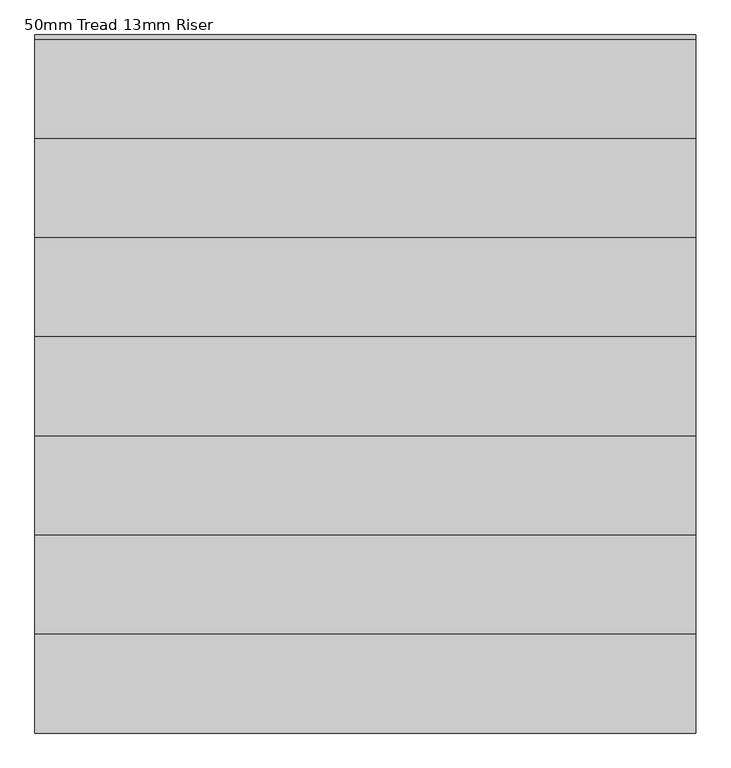
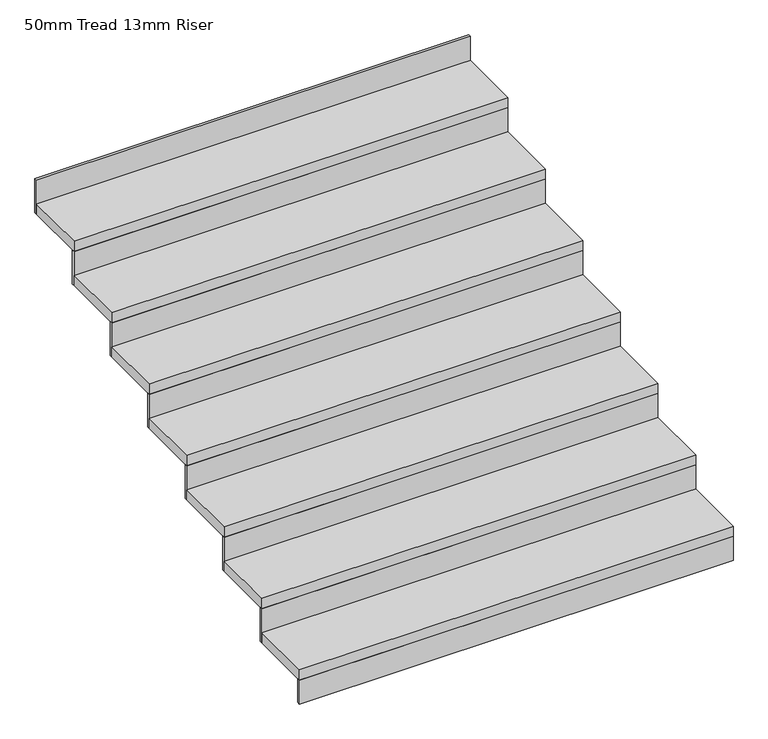
"""IFC4 building model written with IfcOpenShell, lengths in millimetres: stair flight geometry, 50mm Tread 13mm Riser."""

from ifc_helpers import new_model, si_unit, frame, origin, place, context, project, spatial, polyline, outline, extrude, source, transform, mapped, element, save


def stair_flight_50mm_tread_13mm_riser_f0df06f7(model_context):
    return source(origin(), model_context, "Body", "SweptSolid", [
        extrude(outline(polyline([(14700.0002443, 21382.4999999), (14700.0002443, 21369.9999999), (12700.0002443, 21369.9999999), (12700.0002443, 21382.4999999), (14700.0002443, 21382.4999999)])), frame((0.0, 0.0, 26500.0), z_axis=(0.0, 0.0, 1.0), x_axis=(1.0, 0.0, 0.0)), (0.0, 0.0, 1.0), 116.6666667),
        extrude(outline(polyline([(12700.0002443, 21669.9999999), (14700.0002443, 21669.9999999), (14700.0002443, 21369.9999999), (12700.0002443, 21369.9999999), (12700.0002443, 21669.9999999)])), frame((0.0, 0.0, 26616.6666667), z_axis=(0.0, 0.0, 1.0), x_axis=(1.0, 0.0, 0.0)), (0.0, 0.0, 1.0), 50.0),
        extrude(outline(polyline([(14700.0002443, 21682.4999999), (14700.0002443, 21669.9999999), (12700.0002443, 21669.9999999), (12700.0002443, 21682.4999999), (14700.0002443, 21682.4999999)])), frame((0.0, 0.0, 26616.6666667), z_axis=(0.0, 0.0, 1.0), x_axis=(1.0, 0.0, 0.0)), (0.0, 0.0, 1.0), 166.6666667),
        extrude(outline(polyline([(12700.0002443, 21969.9999999), (14700.0002443, 21969.9999999), (14700.0002443, 21669.9999999), (12700.0002443, 21669.9999999), (12700.0002443, 21969.9999999)])), frame((0.0, 0.0, 26783.3333333), z_axis=(0.0, 0.0, 1.0), x_axis=(1.0, 0.0, 0.0)), (0.0, 0.0, 1.0), 50.0),
        extrude(outline(polyline([(14700.0002443, 21982.4999999), (14700.0002443, 21969.9999999), (12700.0002443, 21969.9999999), (12700.0002443, 21982.4999999), (14700.0002443, 21982.4999999)])), frame((0.0, 0.0, 26783.3333333), z_axis=(0.0, 0.0, 1.0), x_axis=(1.0, 0.0, 0.0)), (0.0, 0.0, 1.0), 166.6666667),
        extrude(outline(polyline([(12700.0002443, 22269.9999999), (14700.0002443, 22269.9999999), (14700.0002443, 21969.9999999), (12700.0002443, 21969.9999999), (12700.0002443, 22269.9999999)])), frame((0.0, 0.0, 26950.0), z_axis=(0.0, 0.0, 1.0), x_axis=(1.0, 0.0, 0.0)), (0.0, 0.0, 1.0), 50.0),
        extrude(outline(polyline([(14700.0002443, 22282.4999999), (14700.0002443, 22269.9999999), (12700.0002443, 22269.9999999), (12700.0002443, 22282.4999999), (14700.0002443, 22282.4999999)])), frame((0.0, 0.0, 26950.0), z_axis=(0.0, 0.0, 1.0), x_axis=(1.0, 0.0, 0.0)), (0.0, 0.0, 1.0), 166.6666667),
        extrude(outline(polyline([(12700.0002443, 22569.9999999), (14700.0002443, 22569.9999999), (14700.0002443, 22269.9999999), (12700.0002443, 22269.9999999), (12700.0002443, 22569.9999999)])), frame((0.0, 0.0, 27116.6666667), z_axis=(0.0, 0.0, 1.0), x_axis=(1.0, 0.0, 0.0)), (0.0, 0.0, 1.0), 50.0),
        extrude(outline(polyline([(14700.0002443, 22582.4999999), (14700.0002443, 22569.9999999), (12700.0002443, 22569.9999999), (12700.0002443, 22582.4999999), (14700.0002443, 22582.4999999)])), frame((0.0, 0.0, 27116.6666667), z_axis=(0.0, 0.0, 1.0), x_axis=(1.0, 0.0, 0.0)), (0.0, 0.0, 1.0), 166.6666667),
        extrude(outline(polyline([(12700.0002443, 22869.9999999), (14700.0002443, 22869.9999999), (14700.0002443, 22569.9999999), (12700.0002443, 22569.9999999), (12700.0002443, 22869.9999999)])), frame((0.0, 0.0, 27283.3333333), z_axis=(0.0, 0.0, 1.0), x_axis=(1.0, 0.0, 0.0)), (0.0, 0.0, 1.0), 50.0),
        extrude(outline(polyline([(14700.0002443, 22882.4999999), (14700.0002443, 22869.9999999), (12700.0002443, 22869.9999999), (12700.0002443, 22882.4999999), (14700.0002443, 22882.4999999)])), frame((0.0, 0.0, 27283.3333333), z_axis=(0.0, 0.0, 1.0), x_axis=(1.0, 0.0, 0.0)), (0.0, 0.0, 1.0), 166.6666667),
        extrude(outline(polyline([(12700.0002443, 23169.9999999), (14700.0002443, 23169.9999999), (14700.0002443, 22869.9999999), (12700.0002443, 22869.9999999), (12700.0002443, 23169.9999999)])), frame((0.0, 0.0, 27450.0), z_axis=(0.0, 0.0, 1.0), x_axis=(1.0, 0.0, 0.0)), (0.0, 0.0, 1.0), 50.0),
        extrude(outline(polyline([(14700.0002443, 23182.4999999), (14700.0002443, 23169.9999999), (12700.0002443, 23169.9999999), (12700.0002443, 23182.4999999), (14700.0002443, 23182.4999999)])), frame((0.0, 0.0, 27450.0), z_axis=(0.0, 0.0, 1.0), x_axis=(1.0, 0.0, 0.0)), (0.0, 0.0, 1.0), 166.6666667),
        extrude(outline(polyline([(14700.0002443, 23482.4999999), (14700.0002443, 23469.9999999), (12700.0002443, 23469.9999999), (12700.0002443, 23482.4999999), (14700.0002443, 23482.4999999)])), frame((0.0, 0.0, 27616.6666667), z_axis=(0.0, 0.0, 1.0), x_axis=(1.0, 0.0, 0.0)), (0.0, 0.0, 1.0), 166.6666667),
        extrude(outline(polyline([(12700.0002443, 23469.9999999), (14700.0002443, 23469.9999999), (14700.0002443, 23169.9999999), (12700.0002443, 23169.9999999), (12700.0002443, 23469.9999999)])), frame((0.0, 0.0, 27616.6666667), z_axis=(0.0, 0.0, 1.0), x_axis=(1.0, 0.0, 0.0)), (0.0, 0.0, 1.0), 50.0),
    ])


if __name__ == "__main__":
    model = new_model("IFC4")
    model_context = context("Model", 3, world=origin())
    ifc_project = project(units=[si_unit("LENGTHUNIT", "METRE", prefix="MILLI")], contexts=[model_context])
    site = spatial("IfcSite", under=ifc_project)
    building = spatial("IfcBuilding", under=site)
    placement = place(None, origin())
    stair_flight_50mm_tread_13mm_riser_shape = stair_flight_50mm_tread_13mm_riser_f0df06f7(model_context)
    element("IfcStairFlight", 1, ObjectType="50mm Tread 13mm Riser", at=placement, inside=building, context=model_context, shape_type="MappedRepresentation", body=[
        mapped(stair_flight_50mm_tread_13mm_riser_shape, transform((0.0, 0.0, 0.0), x_axis=(1.0, 0.0, 0.0), y_axis=(0.0, 1.0, 0.0), z_axis=(0.0, 0.0, 1.0))),
    ])
    save(model, "model.ifc")
